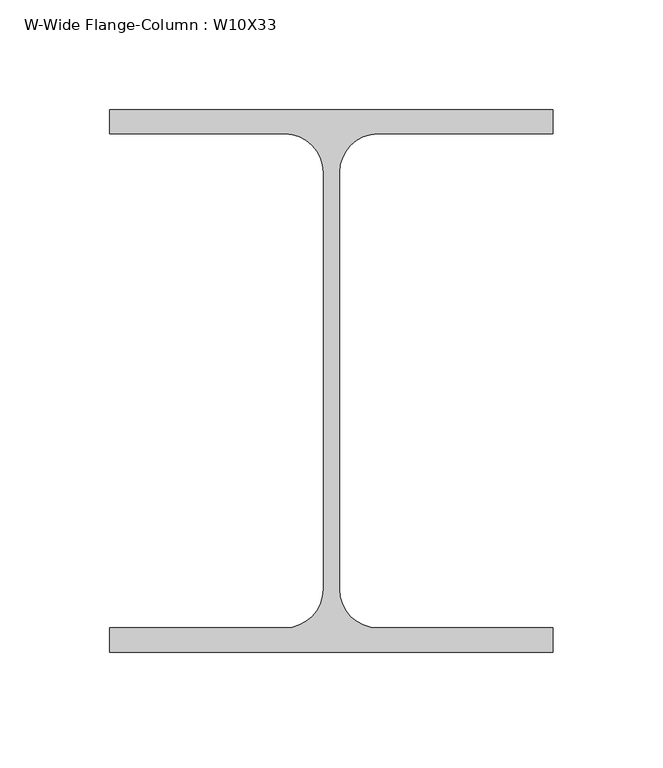
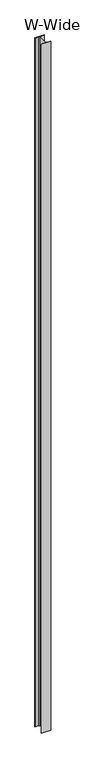
"""IFC4 building model written with IfcOpenShell, lengths in millimetres: column geometry, W-Wide Flange-Column : W10X33."""

from ifc_helpers import new_model, si_unit, point, frame, frame_2d, origin, place, context, project, spatial, polyline, circle_curve, trimmed, segment, composite_curve, outline, extrude, source, transform, mapped, element, save


def w_wide_flange_column_w10x33_42e100d9(model_context):
    return source(origin(), model_context, "Body", "SweptSolid", [
        extrude(outline(composite_curve([segment(polyline([(101.092, 123.571), (101.092, 112.522), (21.209, 112.522)]), True, "CONTINUOUS"), segment(trimmed(circle_curve(frame_2d((21.209, 94.996)), 17.526), [point((21.209, 112.522))], [point((3.683, 94.996))], True, "CARTESIAN"), True, "CONTINUOUS"), segment(polyline([(3.683, 94.996), (3.683, -94.996)]), True, "CONTINUOUS"), segment(trimmed(circle_curve(frame_2d((21.209, -94.996)), 17.526), [point((3.683, -94.996))], [point((21.209, -112.522))], True, "CARTESIAN"), True, "CONTINUOUS"), segment(polyline([(21.209, -112.522), (101.092, -112.522), (101.092, -123.571), (-101.092, -123.571), (-101.092, -112.522), (-21.209, -112.522)]), True, "CONTINUOUS"), segment(trimmed(circle_curve(frame_2d((-21.209, -94.996)), 17.526), [point((-21.209, -112.522))], [point((-3.683, -94.996))], True, "CARTESIAN"), True, "CONTINUOUS"), segment(polyline([(-3.683, -94.996), (-3.683, 94.996)]), True, "CONTINUOUS"), segment(trimmed(circle_curve(frame_2d((-21.209, 94.996)), 17.526), [point((-3.683, 94.996))], [point((-21.209, 112.522))], True, "CARTESIAN"), True, "CONTINUOUS"), segment(polyline([(-21.209, 112.522), (-101.092, 112.522), (-101.092, 123.571), (101.092, 123.571)]), True, "CONTINUOUS")], self_intersect=False)), frame((0.0, 0.0, 8756.65), z_axis=(0.0, 0.0, 1.0), x_axis=(1.0, 0.0, 0.0)), (0.0, 0.0, 1.0), 15982.95),
    ])


if __name__ == "__main__":
    model = new_model("IFC4")
    model_context = context("Model", 3, world=origin())
    ifc_project = project(units=[si_unit("LENGTHUNIT", "METRE", prefix="MILLI")], contexts=[model_context])
    site = spatial("IfcSite", under=ifc_project)
    building = spatial("IfcBuilding", under=site)
    placement = place(None, origin())
    w_wide_flange_column_w10x33_shape = w_wide_flange_column_w10x33_42e100d9(model_context)
    element("IfcColumn", 1, ObjectType="W-Wide Flange-Column : W10X33", at=placement, inside=building, context=model_context, shape_type="MappedRepresentation", body=[
        mapped(w_wide_flange_column_w10x33_shape, transform((0.0, 0.0, 0.0), x_axis=(1.0, 0.0, 0.0), y_axis=(0.0, 1.0, 0.0), z_axis=(0.0, 0.0, 1.0))),
    ])
    save(model, "model.ifc")

# Revit data of these elements
# Type "W-Wide Flange-Column : W10X33"
#   Assembly Code = "B10"
#   W = 33
#   bf = 0' - 7.96"
#   d = 0' - 9.73"
#   k = 0' - 1 1/8"
#   kr = 0' - 0.69"
#   tf = 0' - 0.435"
#   tw = 0' - 0.29"
#   A = 0.0674306 SF
#   Structural Material [instance default] = Steel ASTM A992
# Element 1 (IfcColumn, "W-Wide Flange-Column : W10X33")
#   Materials on its faces: "Steel ASTM A992"
# Materials
#   "Steel ASTM A992": class "Metal", colour RGB 199 199 199, transparency 0, Description = "Structural steel 50ksi", Cost = 0
